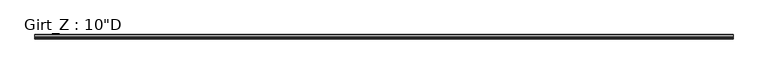
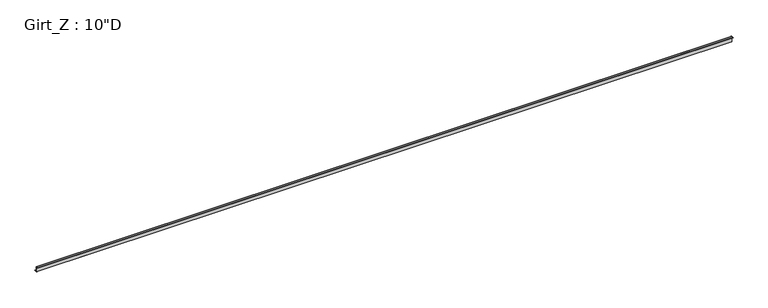
"""IFC4 building model written with IfcOpenShell, lengths in millimetres: beam geometry."""

from ifc_helpers import new_model, si_unit, point, frame, frame_2d, origin, place, context, project, spatial, polyline, circle_curve, trimmed, segment, composite_curve, outline, extrude, source, transform, mapped, element, save


def beam_06492306(model_context):
    return source(origin(), model_context, "Body", "SweptSolid", [
        extrude(outline(composite_curve([segment(polyline([(-77.9859375, 127.0), (-3.3734375, 127.0)]), True, "CONTINUOUS"), segment(trimmed(circle_curve(frame_2d((-3.3734375, 122.2375)), 4.7625), [point((-3.3734375, 127.0))], [point((1.3890625, 122.2375))], False, "CARTESIAN"), True, "CONTINUOUS"), segment(polyline([(1.3890625, 122.2375), (1.3890625, -122.2389339)]), True, "CONTINUOUS"), segment(trimmed(circle_curve(frame_2d((3.3748024, -122.2389339)), 1.9857399), [point((1.3890625, -122.2389339))], [point((3.2694106, -124.221875))], True, "CARTESIAN"), True, "CONTINUOUS"), segment(polyline([(3.2694106, -124.221875), (83.0404765, -124.221875), (94.4528742, -110.621109), (96.5810415, -112.4068534), (84.3359375, -127.0), (-1.3890625, -127.0), (-1.3890625, 122.2381931)]), True, "CONTINUOUS"), segment(trimmed(circle_curve(frame_2d((-3.3741066, 122.2381931)), 1.9850441), [point((-1.3890625, 122.2381931))], [point((-3.3005807, 124.221875))], True, "CARTESIAN"), True, "CONTINUOUS"), segment(polyline([(-3.3005807, 124.221875), (-76.6904765, 124.221875), (-88.1028742, 110.621109), (-90.2310415, 112.4068534), (-77.9859375, 127.0)]), True, "CONTINUOUS")], self_intersect=False)), frame((-15560.6750241, 0.0, 0.0), z_axis=(1.0, 0.0, 0.0), x_axis=(0.0, 1.0, 0.0)), (0.0, 0.0, 1.0), 31121.3500483),
    ])


if __name__ == "__main__":
    model = new_model("IFC4")
    model_context = context("Model", 3, world=origin())
    ifc_project = project(units=[si_unit("LENGTHUNIT", "METRE", prefix="MILLI")], contexts=[model_context])
    site = spatial("IfcSite", under=ifc_project)
    building = spatial("IfcBuilding", under=site)
    placement = place(None, origin())
    beam_shape = beam_06492306(model_context)
    element("IfcBeam", 1, ObjectType="Girt_Z : 10\"D", at=placement, inside=building, context=model_context, shape_type="MappedRepresentation", body=[
        mapped(beam_shape, transform((0.0, 0.0, 0.0), x_axis=(1.0, 0.0, 0.0), y_axis=(0.0, 1.0, 0.0), z_axis=(0.0, 0.0, 1.0))),
    ])
    save(model, "model.ifc")

# Revit data of these elements
# Type "Girt_Z : 10\"D"
#   half leg = 0' - 1 11/16"
#   Web_Thickness = 0' - 0 7/64"
#   Length [instance default] = 10' - 0"
#   Leg_2 = 0' - 3 3/8"
#   Leg_1 = 0' - 3 1/8"
#   Height = 0' - 10"
#   Structural Material [instance default] = none
# Element 1 (IfcBeam, "Girt_Z : 10\"D")
#   Structural Material = STRUCTURAL STEEL - SEE STRUCT. DWGS
#   Materials on its faces: "STRUCTURAL STEEL - SEE STRUCT. DWGS"
# Materials
#   "STRUCTURAL STEEL - SEE STRUCT. DWGS": class "Metal", colour RGB 137 146 153, transparency 0, Description = "Steel, mill finish", Cost = 0
